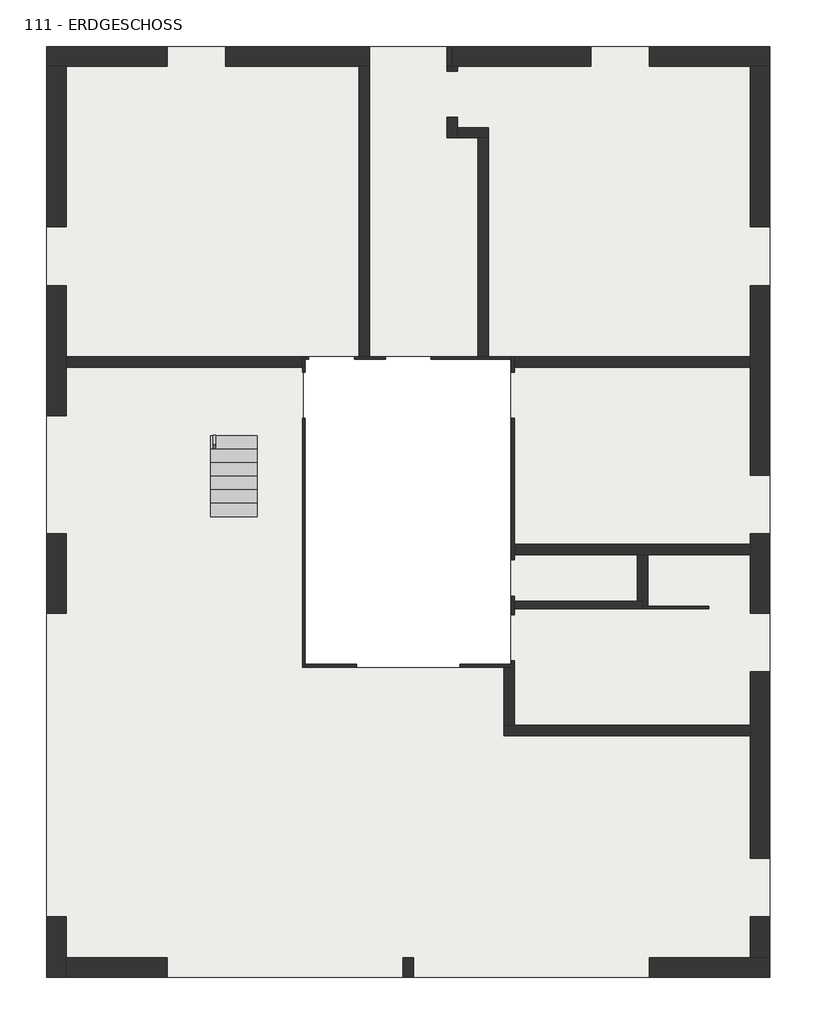
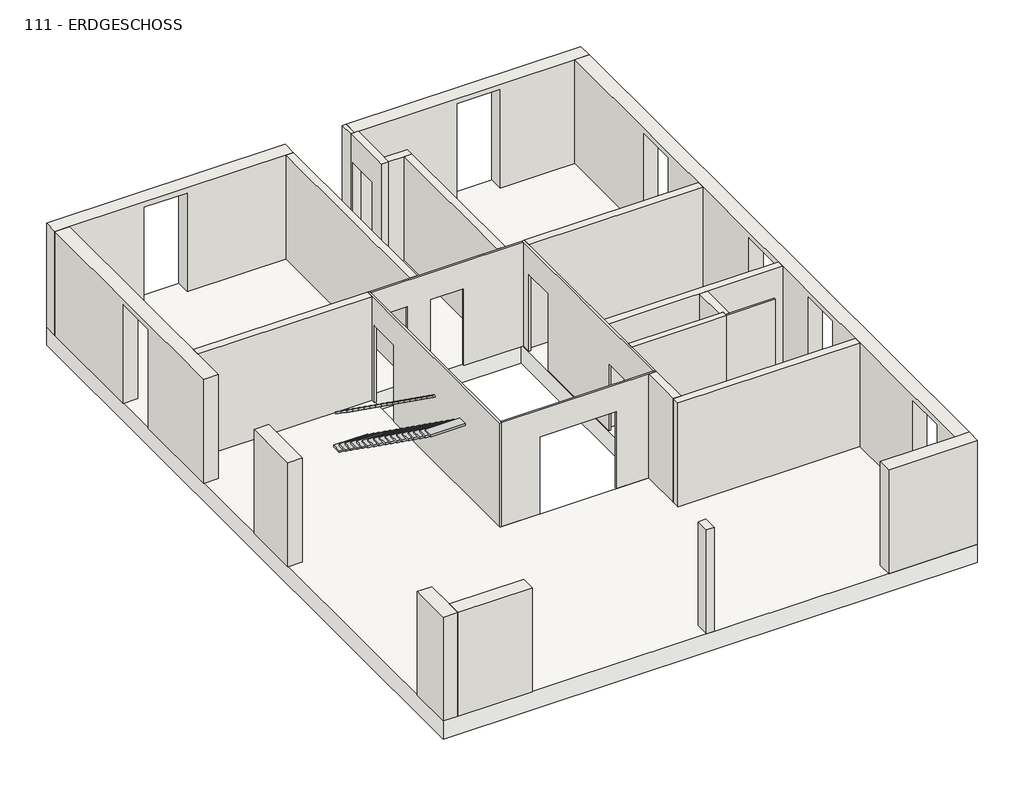
# One storey: 21 walls, 2 stairs, 1 slab.
# Revit data of these elements (continued)
# Element 2 (IfcStair, "  :  ") (continued)
#   IfcGUID = "1$rMRojkz3ThcExnXJjzWS"
#   Phase Created = New Construction
#   Materials on its faces: "*1", "weiss"
# Element 3 (IfcStair, "  92587 :   92587")
#   IFC Predefined Type = "NOTDEFINED"
#   Export to IFC As = "ifcstair"
#   IfcGUID = "2ep3BAGo5B3fqIne1go3vt"
#   Phase Created = New Construction
#   Materials on its faces: "*1", "weiss"
# Element 4 (IfcWall, "Holzwand:1129")
#   Export to IFC As = "ifcwall"
#   IfcGUID = "0DgGR$70f2OvYfKtBoHRz3"
#   NameOverride = "Holzwand"
#   Abrechnungsart = "St"
#   Allright_Bauteil_ID = "0117HWa0000004189"
#   Bezeichnung = "Holzwand"
#   Layer #1:Object Layer Attributes #1:Abrechnungsart = "m²"
#   Layer #1:Object Layer Attributes #1:Allright_Bauteil_ID = "0117Wa 0000004190"
#   Layer #1:Object Layer Attributes #1:Bezeichnung = "Holzwand"
#   Layer #1:Object Layer Attributes #1:Codetext = "HO-WI-HSW\\"
#   Layer #1:Object Layer Attributes #1:Gewerk = "Zimmer- und Holzbauarbeiten"
#   Layer #1:Object Layer Attributes #1:Material = "Holz"
#   Layer #1:Object Layer Attributes #1:Objektname = "Wand"
#   Layer #1:Object Layer Attributes #1:Reference = "Holzwand"
#   Layer #1:Object Layer Attributes #1:Status = "Neubau"
#   MEP Wandtyp = "HO-WA-HSW\\"
#   Objektname = "Gesamtwand"
#   Reference = "Holzwand"
#   Status = "NEW"
#   Top Offset = 0.000 m
#   Base Offset = 0.000 m
#   Unconnected Height = 2.880 m
#   wall height = 2.880 m
#   Layer #1:Object Layer Attributes #1:U-Wert = 0
#   Layer #1:Object Layer Attributes #1:2D Interaktion = yes
#   Layer #1:Object Layer Attributes #1:Außenbauteil = no
#   Layer #1:Object Layer Attributes #1:Brandabschnittsdefinierendes Bauteil = no
#   Layer #1:Object Layer Attributes #1:Brennbares Material = no
#   Layer #1:Object Layer Attributes #1:Raumhohe Wand = yes
#   Layer #1:Object Layer Attributes #1:Tragendes Bauteil = yes
#   ExtendToStructure = yes
#   IsExternal = no
#   LoadBearing = yes
#   Phase Created = New Construction
#   Base Constraint = 111 - ERDGESCHOSS
#   Materials on its faces: "holzschalung"
# Element 5 (IfcWall, "Holzwand:1130")
#   Export to IFC As = "ifcwall"
#   IfcGUID = "3SuUS6DRv0TByZmEwoX91Q"
#   NameOverride = "Holzwand"
#   Abrechnungsart = "St"
#   Allright_Bauteil_ID = "0117HWa0000004204"
#   Bezeichnung = "Holzwand"
#   Layer #1:Object Layer Attributes #1:Abrechnungsart = "m²"
#   Layer #1:Object Layer Attributes #1:Allright_Bauteil_ID = "0117Wa 0000004205"
#   Layer #1:Object Layer Attributes #1:Bezeichnung = "Holzwand"
#   Layer #1:Object Layer Attributes #1:Codetext = "HO-WI-HSW\\"
#   Layer #1:Object Layer Attributes #1:Gewerk = "Zimmer- und Holzbauarbeiten"
#   Layer #1:Object Layer Attributes #1:Material = "Holz"
#   Layer #1:Object Layer Attributes #1:Objektname = "Wand"
#   Layer #1:Object Layer Attributes #1:Reference = "Holzwand"
#   Layer #1:Object Layer Attributes #1:Status = "Neubau"
#   MEP Wandtyp = "HO-WA-HSW\\"
#   Objektname = "Gesamtwand"
#   Reference = "Holzwand"
#   Status = "NEW"
#   Top Offset = 0.000 m
#   Base Offset = 0.000 m
#   Unconnected Height = 2.880 m
#   wall height = 2.880 m
#   Layer #1:Object Layer Attributes #1:U-Wert = 0
#   Layer #1:Object Layer Attributes #1:2D Interaktion = yes
#   Layer #1:Object Layer Attributes #1:Außenbauteil = no
#   Layer #1:Object Layer Attributes #1:Brandabschnittsdefinierendes Bauteil = no
#   Layer #1:Object Layer Attributes #1:Brennbares Material = no
#   Layer #1:Object Layer Attributes #1:Raumhohe Wand = yes
#   Layer #1:Object Layer Attributes #1:Tragendes Bauteil = yes
#   ExtendToStructure = yes
#   IsExternal = no
#   LoadBearing = yes
#   Phase Created = New Construction
#   Base Constraint = 111 - ERDGESCHOSS
#   Materials on its faces: "holzschalung"
# Element 6 (IfcWall, "Holzwand:1131")
#   Export to IFC As = "ifcwall"
#   IfcGUID = "2UeMbe4O5E8gxqwrA1yV32"
#   NameOverride = "Holzwand"
#   Abrechnungsart = "St"
#   Allright_Bauteil_ID = "0117HWa0000624344"
#   Bezeichnung = "Holzwand"
#   Layer #1:Object Layer Attributes #1:Abrechnungsart = "m²"
#   Layer #1:Object Layer Attributes #1:Allright_Bauteil_ID = "0117Wa 0000624345"
#   Layer #1:Object Layer Attributes #1:Bezeichnung = "Holzwand"
#   Layer #1:Object Layer Attributes #1:Codetext = "HO-WI-HSW\\"
#   Layer #1:Object Layer Attributes #1:Gewerk = "Zimmer- und Holzbauarbeiten"
#   Layer #1:Object Layer Attributes #1:Material = "Holz"
#   Layer #1:Object Layer Attributes #1:Objektname = "Wand"
#   Layer #1:Object Layer Attributes #1:Reference = "Holzwand"
#   Layer #1:Object Layer Attributes #1:Status = "Neubau"
#   MEP Wandtyp = "HO-WA-HSW\\"
#   Objektname = "Gesamtwand"
#   Reference = "Holzwand"
#   Status = "NEW"
#   Top Offset = 0.000 m
#   Base Offset = 0.000 m
#   Unconnected Height = 2.880 m
#   wall height = 2.880 m
#   Layer #1:Object Layer Attributes #1:U-Wert = 0
#   Layer #1:Object Layer Attributes #1:2D Interaktion = yes
#   Layer #1:Object Layer Attributes #1:Außenbauteil = no
#   Layer #1:Object Layer Attributes #1:Brandabschnittsdefinierendes Bauteil = no
#   Layer #1:Object Layer Attributes #1:Brennbares Material = no
#   Layer #1:Object Layer Attributes #1:Raumhohe Wand = yes
#   Layer #1:Object Layer Attributes #1:Tragendes Bauteil = yes
#   ExtendToStructure = yes
#   IsExternal = no
#   LoadBearing = yes
#   Phase Created = New Construction
#   Base Constraint = 111 - ERDGESCHOSS
#   Materials on its faces: "holzschalung"
# Element 7 (IfcWall, "Holzwand:1132")
#   Export to IFC As = "ifcwall"
#   IfcGUID = "0dqqUVP3H0ZwAXHPo$n14K"
#   NameOverride = "Holzwand"
#   Abrechnungsart = "St"
#   Allright_Bauteil_ID = "0117HWa0000622592"
#   Bezeichnung = "Holzwand"
#   Layer #1:Object Layer Attributes #1:Abrechnungsart = "m²"
#   Layer #1:Object Layer Attributes #1:Allright_Bauteil_ID = "0117Wa 0000622594"
#   Layer #1:Object Layer Attributes #1:Bezeichnung = "Holzwand"
#   Layer #1:Object Layer Attributes #1:Codetext = "HO-WI-HSW\\"
#   Layer #1:Object Layer Attributes #1:Gewerk = "Zimmer- und Holzbauarbeiten"
#   Layer #1:Object Layer Attributes #1:Material = "Holz"
#   Layer #1:Object Layer Attributes #1:Objektname = "Wand"
#   Layer #1:Object Layer Attributes #1:Reference = "Holzwand"
#   Layer #1:Object Layer Attributes #1:Status = "Neubau"
#   MEP Wandtyp = "HO-WA-HSW\\"
#   Objektname = "Gesamtwand"
#   Reference = "Holzwand"
#   Status = "NEW"
#   Top Offset = 0.000 m
#   Base Offset = 0.000 m
#   Unconnected Height = 2.880 m
#   wall height = 2.880 m
#   Layer #1:Object Layer Attributes #1:U-Wert = 0
#   Layer #1:Object Layer Attributes #1:2D Interaktion = yes
#   Layer #1:Object Layer Attributes #1:Außenbauteil = no
#   Layer #1:Object Layer Attributes #1:Brandabschnittsdefinierendes Bauteil = no
#   Layer #1:Object Layer Attributes #1:Brennbares Material = no
#   Layer #1:Object Layer Attributes #1:Raumhohe Wand = yes
#   Layer #1:Object Layer Attributes #1:Tragendes Bauteil = yes
#   ExtendToStructure = yes
#   IsExternal = no
#   LoadBearing = yes
#   Phase Created = New Construction
#   Base Constraint = 111 - ERDGESCHOSS
#   Materials on its faces: "holzschalung"
# Element 8 (IfcWall, "Holzwand:1133")
#   Export to IFC As = "ifcwall"
#   IfcGUID = "0oSUMut4nB_97re8Y8ood4"
#   NameOverride = "Holzwand"
#   Abrechnungsart = "St"
#   Allright_Bauteil_ID = "0117HWa0000624358"
#   Bezeichnung = "Holzwand"
#   Layer #1:Object Layer Attributes #1:Abrechnungsart = "m²"
#   Layer #1:Object Layer Attributes #1:Allright_Bauteil_ID = "0117Wa 0000624359"
#   Layer #1:Object Layer Attributes #1:Bezeichnung = "Holzwand"
#   Layer #1:Object Layer Attributes #1:Codetext = "HO-WI-HSW\\"
#   Layer #1:Object Layer Attributes #1:Gewerk = "Zimmer- und Holzbauarbeiten"
#   Layer #1:Object Layer Attributes #1:Material = "Holz"
#   Layer #1:Object Layer Attributes #1:Objektname = "Wand"
#   Layer #1:Object Layer Attributes #1:Reference = "Holzwand"
#   Layer #1:Object Layer Attributes #1:Status = "Neubau"
#   MEP Wandtyp = "HO-WA-HSW\\"
#   Objektname = "Gesamtwand"
#   Reference = "Holzwand"
#   Status = "NEW"
#   Top Offset = 0.000 m
#   Base Offset = 0.000 m
#   Unconnected Height = 2.880 m
#   wall height = 2.880 m
#   Layer #1:Object Layer Attributes #1:U-Wert = 0
#   Layer #1:Object Layer Attributes #1:2D Interaktion = yes
#   Layer #1:Object Layer Attributes #1:Außenbauteil = no
#   Layer #1:Object Layer Attributes #1:Brandabschnittsdefinierendes Bauteil = no
#   Layer #1:Object Layer Attributes #1:Brennbares Material = no
#   Layer #1:Object Layer Attributes #1:Raumhohe Wand = yes
#   Layer #1:Object Layer Attributes #1:Tragendes Bauteil = yes
#   ExtendToStructure = yes
#   IsExternal = no
#   LoadBearing = yes
#   Phase Created = New Construction
#   Base Constraint = 111 - ERDGESCHOSS
#   Materials on its faces: "holzschalung"
# Element 9 (IfcWall, "Holzwand:1134")
#   Export to IFC As = "ifcwall"
#   IfcGUID = "1gEmRixYDBmeB186SSf823"
#   NameOverride = "Holzwand"
#   Abrechnungsart = "St"
#   Allright_Bauteil_ID = "0117HWa0000622747"
#   Bezeichnung = "Holzwand"
#   Layer #1:Object Layer Attributes #1:Abrechnungsart = "m²"
#   Layer #1:Object Layer Attributes #1:Allright_Bauteil_ID = "0117Wa 0000622748"
#   Layer #1:Object Layer Attributes #1:Bezeichnung = "Holzwand"
#   Layer #1:Object Layer Attributes #1:Codetext = "HO-WI-HSW\\"
#   Layer #1:Object Layer Attributes #1:Gewerk = "Zimmer- und Holzbauarbeiten"
#   Layer #1:Object Layer Attributes #1:Material = "Holz"
#   Layer #1:Object Layer Attributes #1:Objektname = "Wand"
#   Layer #1:Object Layer Attributes #1:Reference = "Holzwand"
#   Layer #1:Object Layer Attributes #1:Status = "Neubau"
#   MEP Wandtyp = "HO-WA-HSW\\"
#   Objektname = "Gesamtwand"
#   Reference = "Holzwand"
#   Status = "NEW"
#   Top Offset = 0.000 m
#   Base Offset = 0.000 m
#   Unconnected Height = 2.880 m
#   wall height = 2.880 m
#   Layer #1:Object Layer Attributes #1:U-Wert = 0
#   Layer #1:Object Layer Attributes #1:2D Interaktion = yes
#   Layer #1:Object Layer Attributes #1:Außenbauteil = no
#   Layer #1:Object Layer Attributes #1:Brandabschnittsdefinierendes Bauteil = no
#   Layer #1:Object Layer Attributes #1:Brennbares Material = no
#   Layer #1:Object Layer Attributes #1:Raumhohe Wand = yes
#   Layer #1:Object Layer Attributes #1:Tragendes Bauteil = yes
#   ExtendToStructure = yes
#   IsExternal = no
#   LoadBearing = yes
#   Phase Created = New Construction
#   Base Constraint = 111 - ERDGESCHOSS
#   Materials on its faces: "holzschalung"
# Element 10 (IfcWall, "Holzwand:1136")
#   Export to IFC As = "ifcwall"
#   IfcGUID = "151ay_4ln7WvvZWQ8ye2Py"
#   NameOverride = "Holzwand"
#   Abrechnungsart = "St"
#   Allright_Bauteil_ID = "0117HWa0000631785"
#   Bezeichnung = "Holzwand"
#   Layer #1:Object Layer Attributes #1:Abrechnungsart = "m²"
#   Layer #1:Object Layer Attributes #1:Allright_Bauteil_ID = "0117Wa 0000631787"
#   Layer #1:Object Layer Attributes #1:Bezeichnung = "Holzwand"
#   Layer #1:Object Layer Attributes #1:Codetext = "HO-WI-HSW\\"
#   Layer #1:Object Layer Attributes #1:Gewerk = "Zimmer- und Holzbauarbeiten"
#   Layer #1:Object Layer Attributes #1:Material = "Holz"
#   Layer #1:Object Layer Attributes #1:Objektname = "Wand"
#   Layer #1:Object Layer Attributes #1:Reference = "Holzwand"
#   Layer #1:Object Layer Attributes #1:Status = "Neubau"
#   MEP Wandtyp = "HO-WA-HSW\\"
#   Objektname = "Gesamtwand"
#   Reference = "Holzwand"
#   Status = "NEW"
#   Top Offset = 0.000 m
#   Base Offset = 0.000 m
#   Unconnected Height = 2.880 m
#   wall height = 2.880 m
#   Layer #1:Object Layer Attributes #1:U-Wert = 0
#   Layer #1:Object Layer Attributes #1:2D Interaktion = yes
#   Layer #1:Object Layer Attributes #1:Außenbauteil = no
#   Layer #1:Object Layer Attributes #1:Brandabschnittsdefinierendes Bauteil = no
#   Layer #1:Object Layer Attributes #1:Brennbares Material = no
#   Layer #1:Object Layer Attributes #1:Raumhohe Wand = yes
#   Layer #1:Object Layer Attributes #1:Tragendes Bauteil = yes
#   ExtendToStructure = yes
#   IsExternal = no
#   LoadBearing = yes
#   Phase Created = New Construction
#   Base Constraint = 111 - ERDGESCHOSS
#   Materials on its faces: "holzschalung"
# Element 11 (IfcWall, "Holzwand:1137")
#   Export to IFC As = "ifcwall"
#   IfcGUID = "1mJYD8GzX1IA1itJzgwNay"
#   NameOverride = "Holzwand"
#   Abrechnungsart = "St"
#   Allright_Bauteil_ID = "0117HWa0000631790"
#   Bezeichnung = "Holzwand"
#   Layer #1:Object Layer Attributes #1:Abrechnungsart = "m²"
#   Layer #1:Object Layer Attributes #1:Allright_Bauteil_ID = "0117Wa 0000631810"
#   Layer #1:Object Layer Attributes #1:Bezeichnung = "Holzwand"
#   Layer #1:Object Layer Attributes #1:Codetext = "HO-WI-HSW\\"
#   Layer #1:Object Layer Attributes #1:Gewerk = "Zimmer- und Holzbauarbeiten"
#   Layer #1:Object Layer Attributes #1:Material = "Holz"
#   Layer #1:Object Layer Attributes #1:Objektname = "Wand"
#   Layer #1:Object Layer Attributes #1:Reference = "Holzwand"
#   Layer #1:Object Layer Attributes #1:Status = "Neubau"
#   MEP Wandtyp = "HO-WA-HSW\\"
#   Objektname = "Gesamtwand"
#   Reference = "Holzwand"
#   Status = "NEW"
#   Top Offset = 0.000 m
#   Base Offset = 0.000 m
#   Unconnected Height = 2.880 m
#   wall height = 2.880 m
#   Layer #1:Object Layer Attributes #1:U-Wert = 0
#   Layer #1:Object Layer Attributes #1:2D Interaktion = yes
#   Layer #1:Object Layer Attributes #1:Außenbauteil = no
#   Layer #1:Object Layer Attributes #1:Brandabschnittsdefinierendes Bauteil = no
#   Layer #1:Object Layer Attributes #1:Brennbares Material = no
#   Layer #1:Object Layer Attributes #1:Raumhohe Wand = yes
#   Layer #1:Object Layer Attributes #1:Tragendes Bauteil = yes
#   ExtendToStructure = yes
#   IsExternal = no
#   LoadBearing = yes
#   Phase Created = New Construction
#   Base Constraint = 111 - ERDGESCHOSS
#   Materials on its faces: "holzschalung"
# Element 12 (IfcWall, "Holzwand:1139")
#   Export to IFC As = "ifcwall"
#   IfcGUID = "20062VmhnBKxIoOIfzXC3I"
#   NameOverride = "Holzwand"
#   Abrechnungsart = "St"
#   Allright_Bauteil_ID = "0117HWa0000809901"
#   Bezeichnung = "Holzwand"
#   Layer #1:Object Layer Attributes #1:Abrechnungsart = "m²"
#   Layer #1:Object Layer Attributes #1:Allright_Bauteil_ID = "0117Wa 0000809902"
#   Layer #1:Object Layer Attributes #1:Bezeichnung = "Holzwand"
#   Layer #1:Object Layer Attributes #1:Codetext = "HO-WI-HSW\\"
#   Layer #1:Object Layer Attributes #1:Gewerk = "Zimmer- und Holzbauarbeiten"
#   Layer #1:Object Layer Attributes #1:Material = "Holz"
#   Layer #1:Object Layer Attributes #1:Objektname = "Wand"
#   Layer #1:Object Layer Attributes #1:Reference = "Holzwand"
#   Layer #1:Object Layer Attributes #1:Status = "Neubau"
#   MEP Wandtyp = "HO-WA-HSW\\"
#   Objektname = "Gesamtwand"
#   Reference = "Holzwand"
#   Status = "NEW"
#   Top Offset = 0.000 m
#   Base Offset = 0.000 m
#   Unconnected Height = 2.880 m
#   wall height = 2.880 m
#   Layer #1:Object Layer Attributes #1:U-Wert = 0
#   Layer #1:Object Layer Attributes #1:2D Interaktion = yes
#   Layer #1:Object Layer Attributes #1:Außenbauteil = no
#   Layer #1:Object Layer Attributes #1:Brandabschnittsdefinierendes Bauteil = no
#   Layer #1:Object Layer Attributes #1:Brennbares Material = no
#   Layer #1:Object Layer Attributes #1:Raumhohe Wand = yes
#   Layer #1:Object Layer Attributes #1:Tragendes Bauteil = yes
#   ExtendToStructure = yes
#   IsExternal = no
#   LoadBearing = yes
#   Phase Created = New Construction
#   Base Constraint = 111 - ERDGESCHOSS
#   Materials on its faces: "holzschalung"
# Element 13 (IfcWall, "Holzwand:1143")
#   Export to IFC As = "ifcwall"
#   IfcGUID = "051gv9blH6gh$yc7DcDkcn"
#   NameOverride = "Holzwand"
#   Abrechnungsart = "St"
#   Allright_Bauteil_ID = "0117HWa0000966563"
#   Bezeichnung = "Holzwand"
#   Layer #1:Object Layer Attributes #1:Abrechnungsart = "m²"
#   Layer #1:Object Layer Attributes #1:Allright_Bauteil_ID = "0117Wa 0000966564"
#   Layer #1:Object Layer Attributes #1:Codetext = "HO-WI-HSW\\"
#   Layer #1:Object Layer Attributes #1:Gewerk = "Zimmer- und Holzbauarbeiten"
#   Layer #1:Object Layer Attributes #1:Material = "Holz"
#   Layer #1:Object Layer Attributes #1:Objektname = "Wand"
#   Layer #1:Object Layer Attributes #1:Reference = "Holzwand"
#   Layer #1:Object Layer Attributes #1:Status = "Neubau"
#   MEP Wandtyp = "HO-WA-HSW\\"
#   Objektname = "Gesamtwand"
#   Reference = "Holzwand"
#   Status = "NEW"
#   Top Offset = 0.000 m
#   Base Offset = 0.000 m
#   Unconnected Height = 2.880 m
#   wall height = 2.880 m
#   Layer #1:Object Layer Attributes #1:U-Wert = 0
#   Layer #1:Object Layer Attributes #1:2D Interaktion = yes
#   Layer #1:Object Layer Attributes #1:Außenbauteil = no
#   Layer #1:Object Layer Attributes #1:Brandabschnittsdefinierendes Bauteil = no
#   Layer #1:Object Layer Attributes #1:Brennbares Material = no
#   Layer #1:Object Layer Attributes #1:Raumhohe Wand = yes
#   ExtendToStructure = yes
#   IsExternal = no
#   LoadBearing = yes
#   Phase Created = New Construction
#   Base Constraint = 111 - ERDGESCHOSS
#   Materials on its faces: "holzschalung"
# Element 14 (IfcWall, "Holzwand:1144")
#   Export to IFC As = "ifcwall"
#   IfcGUID = "15wLg1nGH8QAa8sQ8toqgz"
#   NameOverride = "Holzwand"
#   Abrechnungsart = "St"
#   Allright_Bauteil_ID = "0117HWa0000631796"
#   Bezeichnung = "Holzwand"
#   Layer #1:Object Layer Attributes #1:Abrechnungsart = "m²"
#   Layer #1:Object Layer Attributes #1:Allright_Bauteil_ID = "0117Wa 0000631798"
#   Layer #1:Object Layer Attributes #1:Codetext = "HO-WI-HSW\\"
#   Layer #1:Object Layer Attributes #1:Gewerk = "Zimmer- und Holzbauarbeiten"
#   Layer #1:Object Layer Attributes #1:Material = "Holz"
#   Layer #1:Object Layer Attributes #1:Objektname = "Wand"
#   Layer #1:Object Layer Attributes #1:Reference = "Holzwand"
#   Layer #1:Object Layer Attributes #1:Status = "Neubau"
#   MEP Wandtyp = "HO-WA-HSW\\"
#   Objektname = "Gesamtwand"
#   Reference = "Holzwand"
#   Status = "NEW"
#   Top Offset = 0.000 m
#   Base Offset = 0.000 m
#   Unconnected Height = 2.880 m
#   wall height = 2.880 m
#   Layer #1:Object Layer Attributes #1:U-Wert = 0
#   Layer #1:Object Layer Attributes #1:2D Interaktion = yes
#   Layer #1:Object Layer Attributes #1:Außenbauteil = no
#   Layer #1:Object Layer Attributes #1:Brandabschnittsdefinierendes Bauteil = no
#   Layer #1:Object Layer Attributes #1:Brennbares Material = no
#   Layer #1:Object Layer Attributes #1:Raumhohe Wand = yes
#   ExtendToStructure = yes
#   IsExternal = no
#   LoadBearing = yes
#   Phase Created = New Construction
#   Base Constraint = 111 - ERDGESCHOSS
#   Materials on its faces: "holzschalung"
# Element 15 (IfcWall, "Holzwand:1145")
#   Export to IFC As = "ifcwall"
#   IfcGUID = "0MES_mtNnA4BdmiBRPnmuy"
#   NameOverride = "Holzwand"
#   Abrechnungsart = "St"
#   Allright_Bauteil_ID = "0117HWa0000631794"
#   Bezeichnung = "Holzwand"
#   Layer #1:Object Layer Attributes #1:Abrechnungsart = "m²"
#   Layer #1:Object Layer Attributes #1:Allright_Bauteil_ID = "0117Wa 0000631809"
#   Layer #1:Object Layer Attributes #1:Codetext = "HO-WI-HSW\\"
#   Layer #1:Object Layer Attributes #1:Gewerk = "Zimmer- und Holzbauarbeiten"
#   Layer #1:Object Layer Attributes #1:Material = "Holz"
#   Layer #1:Object Layer Attributes #1:Objektname = "Wand"
#   Layer #1:Object Layer Attributes #1:Reference = "Holzwand"
#   Layer #1:Object Layer Attributes #1:Status = "Neubau"
#   MEP Wandtyp = "HO-WA-HSW\\"
#   Objektname = "Gesamtwand"
#   Reference = "Holzwand"
#   Status = "NEW"
#   Top Offset = 0.000 m
#   Base Offset = 0.000 m
#   Unconnected Height = 2.880 m
#   wall height = 2.880 m
#   Layer #1:Object Layer Attributes #1:U-Wert = 0
#   Layer #1:Object Layer Attributes #1:2D Interaktion = yes
#   Layer #1:Object Layer Attributes #1:Außenbauteil = no
#   Layer #1:Object Layer Attributes #1:Brandabschnittsdefinierendes Bauteil = no
#   Layer #1:Object Layer Attributes #1:Brennbares Material = no
#   Layer #1:Object Layer Attributes #1:Raumhohe Wand = yes
#   ExtendToStructure = yes
#   IsExternal = no
#   LoadBearing = yes
#   Phase Created = New Construction
#   Base Constraint = 111 - ERDGESCHOSS
#   Materials on its faces: "holzschalung"
# Element 16 (IfcWall, " :1146")
#   Export to IFC As = "ifcwall"
#   IfcGUID = "223fSHhSnDihUf5KQvJ9lc"
#   NameOverride = " "
#   Abrechnungsart = "m³"
#   Allright_Bauteil_ID = "0117HWa0000000025"
#   Layer #1:Object Layer Attributes #1:Abrechnungsart = "m²"
#   Layer #1:Object Layer Attributes #1:Allright_Bauteil_ID = "0117Wa 0000000040"
#   Layer #1:Object Layer Attributes #1:Gewerk = "Zimmer- und Holzbauarbeiten"
#   Layer #1:Object Layer Attributes #1:Material = "k.Ausw."
#   Layer #1:Object Layer Attributes #1:Objektname = "Wand"
#   Layer #1:Object Layer Attributes #1:Status = "Neubau"
#   MEP Wandtyp = "HO-WA-HSW\\"
#   Objektname = "Gesamtwand"
#   Top Offset = 0.000 m
#   Base Offset = 0.000 m
#   Unconnected Height = 2.880 m
#   wall height = 2.880 m
#   Layer #1:Object Layer Attributes #1:2D Interaktion = yes
#   Phase Created = New Construction
#   Base Constraint = 111 - ERDGESCHOSS
#   Materials on its faces: "glas"
# Element 17 (IfcWall, " :1147")
#   Export to IFC As = "ifcwall"
#   IfcGUID = "3AVFvXaUr74xxKMKcP3Kgj"
#   NameOverride = " "
#   Abrechnungsart = "m³"
#   Allright_Bauteil_ID = "0117HWa0000000032"
#   Layer #1:Object Layer Attributes #1:Abrechnungsart = "m²"
#   Layer #1:Object Layer Attributes #1:Allright_Bauteil_ID = "0117Wa 0000000038"
#   Layer #1:Object Layer Attributes #1:Gewerk = "Zimmer- und Holzbauarbeiten"
#   Layer #1:Object Layer Attributes #1:Material = "k.Ausw."
#   Layer #1:Object Layer Attributes #1:Objektname = "Wand"
#   Layer #1:Object Layer Attributes #1:Status = "Neubau"
#   MEP Wandtyp = "HO-WA-HSW\\"
#   Objektname = "Gesamtwand"
#   Top Offset = 0.000 m
#   Base Offset = 0.000 m
#   Unconnected Height = 2.880 m
#   wall height = 2.880 m
#   Layer #1:Object Layer Attributes #1:2D Interaktion = yes
#   Phase Created = New Construction
#   Base Constraint = 111 - ERDGESCHOSS
#   Materials on its faces: "glas"
# Element 18 (IfcWall, " :1148")
#   Export to IFC As = "ifcwall"
#   IfcGUID = "0IU0EKF2HFggyClhwVCNCR"
#   NameOverride = " "
#   Abrechnungsart = "m³"
#   Allright_Bauteil_ID = "0117HWa0000000023"
#   Layer #1:Object Layer Attributes #1:Abrechnungsart = "m²"
#   Layer #1:Object Layer Attributes #1:Allright_Bauteil_ID = "0117Wa 0000000042"
#   Layer #1:Object Layer Attributes #1:Gewerk = "Zimmer- und Holzbauarbeiten"
#   Layer #1:Object Layer Attributes #1:Material = "k.Ausw."
#   Layer #1:Object Layer Attributes #1:Objektname = "Wand"
#   Layer #1:Object Layer Attributes #1:Status = "Neubau"
#   MEP Wandtyp = "HO-WA-HSW\\"
#   Objektname = "Gesamtwand"
#   Top Offset = 0.000 m
#   Base Offset = 0.000 m
#   Unconnected Height = 2.880 m
#   wall height = 2.880 m
#   Layer #1:Object Layer Attributes #1:2D Interaktion = yes
#   Phase Created = New Construction
#   Base Constraint = 111 - ERDGESCHOSS
#   Materials on its faces: "glas"
# Element 19 (IfcWall, " :1149")
#   Export to IFC As = "ifcwall"
#   IfcGUID = "1POtITosf6HgDrOtLssfSq"
#   NameOverride = " "
#   Abrechnungsart = "m³"
#   Allright_Bauteil_ID = "0117HWa0000000029"
#   Layer #1:Object Layer Attributes #1:Abrechnungsart = "m²"
#   Layer #1:Object Layer Attributes #1:Allright_Bauteil_ID = "0117Wa 0000000036"
#   Layer #1:Object Layer Attributes #1:Gewerk = "Zimmer- und Holzbauarbeiten"
#   Layer #1:Object Layer Attributes #1:Material = "k.Ausw."
#   Layer #1:Object Layer Attributes #1:Objektname = "Wand"
#   Layer #1:Object Layer Attributes #1:Status = "Neubau"
#   MEP Wandtyp = "HO-WA-HSW\\"
#   Objektname = "Gesamtwand"
#   Top Offset = 0.000 m
#   Base Offset = 0.000 m
#   Unconnected Height = 2.880 m
#   wall height = 2.880 m
#   Layer #1:Object Layer Attributes #1:2D Interaktion = yes
#   Phase Created = New Construction
#   Base Constraint = 111 - ERDGESCHOSS
#   Materials on its faces: "glas"
# Element 20 (IfcWall, "1141 Aussenwand")
#   Export to IFC As = "ifcwall"
#   IfcGUID = "16fmitl_v098kiyuUgdxdb"
#   NameOverride = " "
#   Abrechnungsart = "m³"
#   Allright_Bauteil_ID = "0117HWa0000000007"
#   Layer #1:Object Layer Attributes #1:Abrechnungsart = "m²"
#   Layer #1:Object Layer Attributes #1:Allright_Bauteil_ID = "0117Wa 0000000022"
#   Layer #1:Object Layer Attributes #1:Gewerk = "Zimmer- und Holzbauarbeiten"
#   Layer #1:Object Layer Attributes #1:Material = "k.Ausw."
#   Layer #1:Object Layer Attributes #1:Objektname = "Wand"
#   Layer #1:Object Layer Attributes #1:Status = "Neubau"
#   MEP Wandtyp = "HO-WA-HSW\\"
#   Objektname = "Gesamtwand"
#   Top Offset = 0.000 m
#   Base Offset = 0.000 m
#   Unconnected Height = 2.880 m
#   wall height = 2.880 m
#   Layer #1:Object Layer Attributes #1:2D Interaktion = yes
#   Layer #1:Object Layer Attributes #1:Tragendes Bauteil = no
#   Phase Created = New Construction
#   Base Constraint = 111 - ERDGESCHOSS
#   Materials on its faces: "holzschalung"
# Element 21 (IfcWall, "1141 Aussenwand")
#   Export to IFC As = "ifcwall"
#   IfcGUID = "2XS7ZdlbfC6vteejEkE541"
#   NameOverride = " "
#   Abrechnungsart = "m³"
#   Allright_Bauteil_ID = "0117HWa0000000014"
#   Layer #1:Object Layer Attributes #1:Abrechnungsart = "m²"
#   Layer #1:Object Layer Attributes #1:Allright_Bauteil_ID = "0117Wa 0000000055"
#   Layer #1:Object Layer Attributes #1:Gewerk = "Zimmer- und Holzbauarbeiten"
#   Layer #1:Object Layer Attributes #1:Material = "k.Ausw."
#   Layer #1:Object Layer Attributes #1:Objektname = "Wand"
#   Layer #1:Object Layer Attributes #1:Status = "Neubau"
#   MEP Wandtyp = "HO-WA-HSW\\"
#   Objektname = "Gesamtwand"
#   Top Offset = 0.000 m
#   Base Offset = 0.000 m
#   Unconnected Height = 2.880 m
#   wall height = 2.880 m
#   Layer #1:Object Layer Attributes #1:2D Interaktion = yes
#   Phase Created = New Construction
#   Base Constraint = 111 - ERDGESCHOSS
#   Materials on its faces: "holzschalung"
# Element 22 (IfcWall, "1141 Aussenwand")
#   Export to IFC As = "ifcwall"
#   IfcGUID = "1yfNVxTDD71fm3F6cC1BDU"
#   Comments = "EG Sued"
#   Mark = "EG Sued"
#   NameOverride = " "
#   Abrechnungsart = "m³"
#   Allright_Bauteil_ID = "0117HWa0000000045"
#   Layer #1:Object Layer Attributes #1:Abrechnungsart = "m²"
#   Layer #1:Object Layer Attributes #1:Allright_Bauteil_ID = "0117Wa 0000000050"
#   Layer #1:Object Layer Attributes #1:Gewerk = "Zimmer- und Holzbauarbeiten"
#   Layer #1:Object Layer Attributes #1:Material = "k.Ausw."
#   Layer #1:Object Layer Attributes #1:Objektname = "Wand"
#   Layer #1:Object Layer Attributes #1:Status = "Neubau"
#   MEP Wandtyp = "HO-WA-HSW\\"
#   Objektname = "Gesamtwand"
#   Top Offset = 0.000 m
#   Base Offset = 0.000 m
#   Unconnected Height = 2.880 m
#   wall height = 2.880 m
#   Layer #1:Object Layer Attributes #1:2D Interaktion = yes
#   Layer #1:Object Layer Attributes #1:Tragendes Bauteil = no
#   Phase Created = New Construction
#   Base Constraint = 111 - ERDGESCHOSS
#   Materials on its faces: "holzschalung"
# Element 23 (IfcWall, "1141 Aussenwand")
#   Export to IFC As = "ifcwall"
#   IfcGUID = "3nAIkQEX5F5fkLRNdJoOx5"
#   NameOverride = " "
#   Abrechnungsart = "m³"
#   Allright_Bauteil_ID = "0117HWa0000000016"
#   Layer #1:Object Layer Attributes #1:Abrechnungsart = "m²"
#   Layer #1:Object Layer Attributes #1:Allright_Bauteil_ID = "0117Wa 0000000020"
#   Layer #1:Object Layer Attributes #1:Gewerk = "Zimmer- und Holzbauarbeiten"
#   Layer #1:Object Layer Attributes #1:Material = "k.Ausw."
#   Layer #1:Object Layer Attributes #1:Objektname = "Wand"
#   Layer #1:Object Layer Attributes #1:Status = "Neubau"
#   MEP Wandtyp = "HO-WA-HSW\\"
#   Objektname = "Gesamtwand"
#   Top Offset = 0.000 m
#   Base Offset = 0.000 m
#   Unconnected Height = 2.880 m
#   wall height = 2.880 m
#   Layer #1:Object Layer Attributes #1:2D Interaktion = yes
#   Phase Created = New Construction
#   Base Constraint = 111 - ERDGESCHOSS
#   Materials on its faces: "holzschalung"
# Element 24 (IfcWall, "1141 Aussenwand")
#   Export to IFC As = "ifcwall"
#   IfcGUID = "2fwekwcCDDz9jpXxCat4j4"
#   NameOverride = " "
#   Abrechnungsart = "m³"
#   Allright_Bauteil_ID = "0117HWa0000622659"
#   Layer #1:Object Layer Attributes #1:Abrechnungsart = "m²"
#   Layer #1:Object Layer Attributes #1:Allright_Bauteil_ID = "0117Wa 0000622663"
#   Layer #1:Object Layer Attributes #1:Gewerk = "Zimmer- und Holzbauarbeiten"
#   Layer #1:Object Layer Attributes #1:Material = "k.Ausw."
#   Layer #1:Object Layer Attributes #1:Objektname = "Wand"
#   Layer #1:Object Layer Attributes #1:Status = "Neubau"
#   MEP Wandtyp = "HO-WA-HSW\\"
#   Objektname = "Gesamtwand"
#   Top Offset = 0.000 m
#   Base Offset = 0.000 m
#   Unconnected Height = 2.880 m
#   wall height = 2.880 m
#   Layer #1:Object Layer Attributes #1:2D Interaktion = yes
#   Phase Created = New Construction
#   Base Constraint = 111 - ERDGESCHOSS
#   Materials on its faces: "holzschalung"
# Materials
#   "holzschalung": class "Unassigned", colour RGB 128 128 128, transparency 0
#   "glas": class "Unassigned", colour RGB 250 253 254, transparency 0.95
#   "Default Floor": class "Miscellaneous", colour RGB 128 128 128, transparency 0, Cost = 0
#   "*1": class "Unassigned", colour RGB 175 175 175, transparency 0
#   "weiss": class "Unassigned", colour RGB 255 255 255, transparency 0
# Room at (3137.096, 14025) mm, phase "New Construction", upper offset 2.880 m, lower offset 0.000 m
#   Export to IFC As = "ifcspace"
#   IfcGUID = "3qaIoGBT54VxUGXoZd$XKS"
#   Comments = ""
#   Number = "22"
#   Name = "Zimmer 4"
#   Abrechnungsart = "m²"
#   Allright_Bauteil_ID = "0117Rau0000621569"
#   Objektname = "Raum"
#   Status = "Neubau"
#   Flächenart_DIN277 = "N"
#   Flächenart_Wohnfläche = "WO"
#   Nutzungsart_Din277 = "NUF"
#   Ortscode_Geschoßbezeichnung = "EG"
#   Raumumschließung = "R"
#   Faktor_DIN277 = 1
#   Faktor_Wohnfläche_Raum = 1
#   BauNVO_Anrechnung_auf_GF = 0
#   BauNVO_Anrechnung_auf_GR = 0
#   Raum unter Treppe (Wohnfl erst ab 2m) = 0
# Room at (6039.465, 7638.569) mm, phase "New Construction", upper offset 2.880 m, lower offset 0.000 m
#   Export to IFC As = "ifcspace"
#   IfcGUID = "2MQ3UCf617TP_Fjr$SAPtE"
#   Comments = ""
#   Number = "23"
#   Name = "Küche/Gemeinschftsraum"
#   Abrechnungsart = "m²"
#   Allright_Bauteil_ID = "0117Rau0000803402"
#   Objektname = "Raum"
#   Status = "Neubau"
#   Flächenart_DIN277 = "N"
#   Flächenart_Wohnfläche = "WO"
#   Nutzungsart_Din277 = "NUF"
#   Ortscode_Geschoßbezeichnung = "EG"
#   Raumumschließung = "R"
#   Faktor_DIN277 = 1
#   Faktor_Wohnfläche_Raum = 1
#   BauNVO_Anrechnung_auf_GF = 0
#   BauNVO_Anrechnung_auf_GR = 0
#   Raum unter Treppe (Wohnfl erst ab 2m) = 0
# Room at (11299.269, 9275) mm, phase "New Construction", upper offset 2.880 m, lower offset 0.000 m
#   Export to IFC As = "ifcspace"
#   IfcGUID = "2TPXanZZfDXhq6h4AZ3bl4"
#   Comments = ""
#   Number = "24"
#   Name = "WC"
#   Abrechnungsart = "m²"
#   Allright_Bauteil_ID = "0117Rau0000977083"
#   Objektname = "Raum"
#   Status = "Neubau"
#   Flächenart_DIN277 = "N"
#   Flächenart_Wohnfläche = "WO"
#   Nutzungsart_Din277 = "NUF"
#   Ortscode_Geschoßbezeichnung = "EG"
#   Raumumschließung = "R"
#   Faktor_DIN277 = 1
#   Faktor_Wohnfläche_Raum = 1
#   BauNVO_Anrechnung_auf_GF = 0
#   BauNVO_Anrechnung_auf_GR = 0
#   Raum unter Treppe (Wohnfl erst ab 2m) = 0
# Room at (11985.707, 11637.5) mm, phase "New Construction", upper offset 2.880 m, lower offset 0.000 m
#   Export to IFC As = "ifcspace"
#   IfcGUID = "3CGOY14EPF9QduD$DK3w2B"
#   Comments = ""
#   Number = "25"
#   Name = "Gästezimmer"
#   Abrechnungsart = "m²"
#   Allright_Bauteil_ID = "0117Rau0000803284"
#   Objektname = "Raum"
#   Status = "Neubau"
#   Flächenart_DIN277 = "N"
#   Flächenart_Wohnfläche = "WO"
#   Nutzungsart_Din277 = "NUF"
#   Ortscode_Geschoßbezeichnung = "EG"
#   Raumumschließung = "R"
#   Faktor_DIN277 = 1
#   Faktor_Wohnfläche_Raum = 1
#   BauNVO_Anrechnung_auf_GF = 0
#   BauNVO_Anrechnung_auf_GR = 0
#   Raum unter Treppe (Wohnfl erst ab 2m) = 0
# Room at (11985.707, 7550) mm, phase "New Construction", upper offset 2.880 m, lower offset 0.000 m
#   Export to IFC As = "ifcspace"
#   IfcGUID = "02maTnz2DBERNGgUPrume0"
#   Comments = ""
#   Number = "26"
#   Name = "Bad"
#   Abrechnungsart = "m²"
#   Allright_Bauteil_ID = "0117Rau0000976666"
#   Objektname = "Raum"
#   Status = "Neubau"
#   Flächenart_DIN277 = "N"
#   Flächenart_Wohnfläche = "WO"
#   Nutzungsart_Din277 = "NUF"
#   Ortscode_Geschoßbezeichnung = "EG"
#   Raumumschließung = "R"
#   Faktor_DIN277 = 1
#   Faktor_Wohnfläche_Raum = 1
#   BauNVO_Anrechnung_auf_GF = 0
#   BauNVO_Anrechnung_auf_GR = 0
#   Raum unter Treppe (Wohnfl erst ab 2m) = 0
# Room at (11231.282, 16360) mm, phase "New Construction", upper offset 2.880 m, lower offset 0.000 m
#   Export to IFC As = "ifcspace"
#   IfcGUID = "0kP5NctjTDWOIqk7IPhDg_"
#   Comments = ""
#   Number = "27"
#   Name = "Hauswirtschaft/Technik"
#   Abrechnungsart = "m²"
#   Allright_Bauteil_ID = "0117Rau0000803301"
#   Objektname = "Raum"
#   Status = "Neubau"
#   Flächenart_DIN277 = "N"
#   Flächenart_Wohnfläche = "WO"
#   Nutzungsart_Din277 = "NUF"
#   Ortscode_Geschoßbezeichnung = "EG"
#   Raumumschließung = "R"
#   Faktor_DIN277 = 1
#   Faktor_Wohnfläche_Raum = 1
#   BauNVO_Anrechnung_auf_GF = 0
#   BauNVO_Anrechnung_auf_GR = 0
#   Raum unter Treppe (Wohnfl erst ab 2m) = 0
# Room at (3661.282, 16835) mm, phase "New Construction", upper offset 2.880 m, lower offset 0.000 m
#   Export to IFC As = "ifcspace"
#   IfcGUID = "3M1IJah$b3_wuZJx3ntBW$"
#   Comments = ""
#   Number = "28"
#   Name = "Zimmer 1"
#   Abrechnungsart = "m²"
#   Allright_Bauteil_ID = "0117Rau0000782817"
#   Objektname = "Raum"
#   Status = "Neubau"
#   Flächenart_DIN277 = "N"
#   Flächenart_Wohnfläche = "WO"
#   Nutzungsart_Din277 = "NUF"
#   Ortscode_Geschoßbezeichnung = "EG"
#   Raumumschließung = "R"
#   Faktor_DIN277 = 1
#   Faktor_Wohnfläche_Raum = 1
#   BauNVO_Anrechnung_auf_GF = 0
#   BauNVO_Anrechnung_auf_GR = 0
#   Raum unter Treppe (Wohnfl erst ab 2m) = 0
# Room at (8800, 15315.574) mm, phase "New Construction", upper offset 2.880 m, lower offset 0.000 m
#   Export to IFC As = "ifcspace"
#   IfcGUID = "1ARQU3MDf1mR6c3l7jOZM5"
#   Comments = ""
#   Number = "29"
#   Name = "Flur"
#   Abrechnungsart = "m²"
#   Allright_Bauteil_ID = "0117Rau0000625508"
#   Objektname = "Raum"
#   Status = "Neubau"
#   Flächenart_DIN277 = "N"
#   Flächenart_Wohnfläche = "WO"
#   Nutzungsart_Din277 = "NUF"
#   Ortscode_Geschoßbezeichnung = "EG"
#   Raumumschließung = "R"
#   Faktor_DIN277 = 1
#   Faktor_Wohnfläche_Raum = 1
#   BauNVO_Anrechnung_auf_GF = 0
#   BauNVO_Anrechnung_auf_GR = 0
#   Raum unter Treppe (Wohnfl erst ab 2m) = 0
